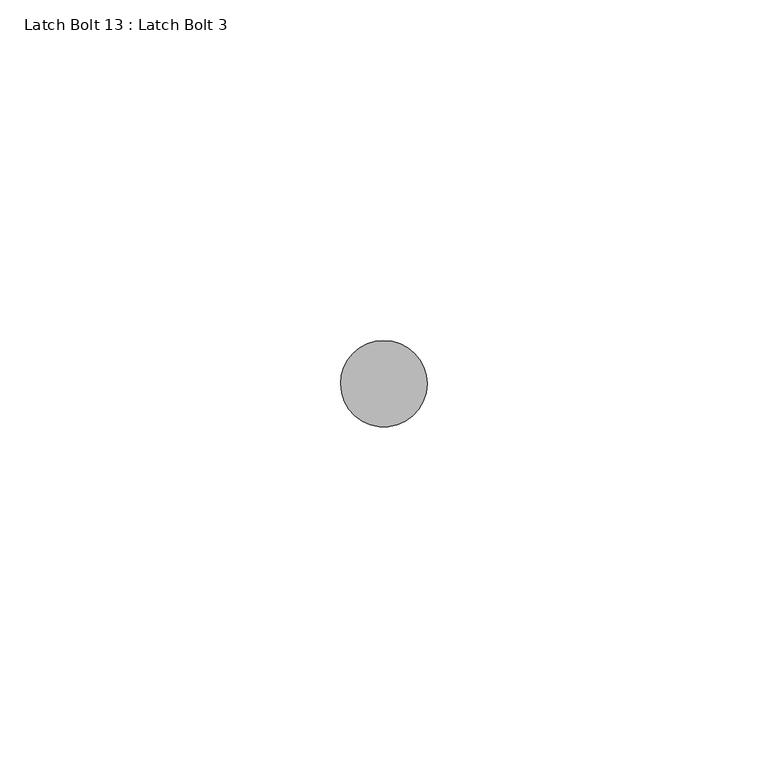
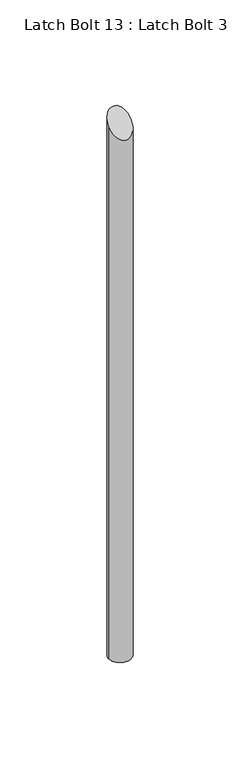
"""IFC4 building model written with IfcOpenShell, lengths in millimetres: proxy geometry, Latch Bolt 13 : Latch Bolt 3."""

import ifcopenshell
import ifcopenshell.guid

model = None  # the IFC model being written
_history = None  # IfcOwnerHistory: only IFC2X3 demands one
_inside = {}  # id of a spatial element -> (the spatial element, [elements in it])
_under = {}  # id of a project, library or spatial element -> (it, [spatial elements below it])
_declared = {}  # id of a project -> (the project, [libraries it declares])
_typed = {}  # id of a type object -> (the type object, [elements of that type])
_made_of = {}  # id of a material, layer set ... -> (it, [elements and type objects made of it])


def new_model(schema):
    """Start an empty IFC model of exactly this schema.

    Asked for "IFC4X3", IfcOpenShell would pick the latest addendum, in which some entities
    have other attributes; the version numbers below select the first issue.
    IFC2X3 requires an IfcOwnerHistory on every rooted entity: one is made here for all.
    """
    global model, _history
    if schema == "IFC4X3":
        model = ifcopenshell.file(schema_version=(4, 3, 0, 0))
    else:
        model = ifcopenshell.file(schema=schema)
    _inside.clear()
    _under.clear()
    _declared.clear()
    _typed.clear()
    _made_of.clear()
    _history = None
    if model.schema == "IFC2X3":
        org = make("IfcOrganization", Name="unknown")
        user = make(
            "IfcPersonAndOrganization",
            ThePerson=make("IfcPerson", FamilyName="unknown"),
            TheOrganization=org,
        )
        app = make(
            "IfcApplication",
            ApplicationDeveloper=org,
            Version="unknown",
            ApplicationFullName="unknown",
            ApplicationIdentifier="unknown",
        )
        _history = make(
            "IfcOwnerHistory",
            OwningUser=user,
            OwningApplication=app,
            ChangeAction="ADDED",
            CreationDate=0,
        )
    return model


def make(cls, **values):
    """One entity of the class cls with the attributes given. An attribute that is None is left unset."""
    return model.create_entity(
        cls, **{name: value for name, value in values.items() if value is not None}
    )


def rooted(cls, **values):
    """An entity with a GlobalId (a new one), such as an element, a storey or a relation."""
    return make(cls, GlobalId=ifcopenshell.guid.new(), OwnerHistory=_history, **values)


def si_unit(unit_type, name, prefix=None):
    """IfcSIUnit, for example si_unit("LENGTHUNIT", "METRE", prefix="MILLI")."""
    return make("IfcSIUnit", UnitType=unit_type, Prefix=prefix, Name=name)


def assignment(units):
    """IfcUnitAssignment: the units of a project."""
    return None if units is None else make("IfcUnitAssignment", Units=units)


def point(xyz):
    """IfcCartesianPoint."""
    return None if xyz is None else make("IfcCartesianPoint", Coordinates=xyz)


def direction(xyz):
    """IfcDirection."""
    return None if xyz is None else make("IfcDirection", DirectionRatios=xyz)


def frame(location, z_axis=None, x_axis=None):
    """IfcAxis2Placement3D, a coordinate frame: its origin and axes. An axis left out is left unset."""
    return make(
        "IfcAxis2Placement3D",
        Location=point(location),
        Axis=direction(z_axis),
        RefDirection=direction(x_axis),
    )


def origin():
    """The frame at (0, 0, 0) with its axes left unset."""
    return frame((0.0, 0.0, 0.0))


def place(relative_to, where):
    """IfcLocalPlacement: puts the frame where relative to a parent placement (None: the world)."""
    return make(
        "IfcLocalPlacement", PlacementRelTo=relative_to, RelativePlacement=where
    )


def context(
    kind, dimensions, precision=None, world=None, true_north=None, identifier=None
):
    """IfcGeometricRepresentationContext, for example the 3D "Model" context."""
    return make(
        "IfcGeometricRepresentationContext",
        ContextIdentifier=identifier,
        ContextType=kind,
        CoordinateSpaceDimension=dimensions,
        Precision=precision,
        WorldCoordinateSystem=world,
        TrueNorth=true_north,
    )


def project(units=None, contexts=None):
    """IfcProject with its units and contexts."""
    return rooted(
        "IfcProject",
        Name="project",
        RepresentationContexts=contexts,
        UnitsInContext=assignment(units),
    )


def spatial(cls, under=None, at=None, **own):
    """A site, building, storey or space (cls), placed at a placement, below another one or the project."""
    s = rooted(cls, ObjectPlacement=at, **own)
    if under is not None:
        _under.setdefault(under.id(), (under, []))[1].append(s)
    return s


def circle_curve(where, radius):
    """IfcCircle in the frame where."""
    return make("IfcCircle", Position=where, Radius=radius)


def ellipse_curve(where, semi_axis1, semi_axis2):
    """IfcEllipse in the frame where."""
    return make(
        "IfcEllipse", Position=where, SemiAxis1=semi_axis1, SemiAxis2=semi_axis2
    )


def shape(context_of_items, identifier, shape_type, items):
    """IfcShapeRepresentation: the items that make up one representation, for example the "Body"."""
    return make(
        "IfcShapeRepresentation",
        ContextOfItems=context_of_items,
        RepresentationIdentifier=identifier,
        RepresentationType=shape_type,
        Items=items,
    )


def source(mapping_origin, context_of_items, identifier, shape_type, items):
    """IfcRepresentationMap: a shape defined once, which mapped items show again and again."""
    return make(
        "IfcRepresentationMap",
        MappingOrigin=mapping_origin,
        MappedRepresentation=shape(context_of_items, identifier, shape_type, items),
    )


def transform(
    local_origin,
    x_axis=None,
    y_axis=None,
    z_axis=None,
    scale=None,
    scale2=None,
    scale3=None,
    uniform=True,
):
    """IfcCartesianTransformationOperator3D, or its non-uniform kind. x_axis, y_axis, z_axis: its Axis1, 2, 3."""
    if uniform:
        return make(
            "IfcCartesianTransformationOperator3D",
            Axis1=direction(x_axis),
            Axis2=direction(y_axis),
            LocalOrigin=point(local_origin),
            Scale=scale,
            Axis3=direction(z_axis),
        )
    return make(
        "IfcCartesianTransformationOperator3DnonUniform",
        Axis1=direction(x_axis),
        Axis2=direction(y_axis),
        LocalOrigin=point(local_origin),
        Scale=scale,
        Axis3=direction(z_axis),
        Scale2=scale2,
        Scale3=scale3,
    )


def mapped(mapping_source, mapping_target):
    """IfcMappedItem: shows the shape of a source again, moved by a transform."""
    return make(
        "IfcMappedItem", MappingSource=mapping_source, MappingTarget=mapping_target
    )


def made_of(thing, what):
    """Note that an element or type object is made of a material, layer set ...; save() writes the relation."""
    if what is not None:
        _made_of.setdefault(what.id(), (what, []))[1].append(thing)
    return thing


def element(
    cls,
    number,
    at=None,
    inside=None,
    cuts=None,
    type_object=None,
    material=None,
    context=None,
    identifier="Body",
    shape_type=None,
    held_by="IfcProductDefinitionShape",
    body=None,
    shapes=None,
    **own,
):
    """One element of the class cls, such as IfcWall. Its Tag is "e" and its number.

    at: its placement. inside: the storey or other place that contains it. cuts: it is an
    opening in that element (IfcRelVoidsElement). A single representation is given by context,
    identifier, shape_type and body (its items); several are given by shapes. held_by: the class
    of the entity that holds the representations. save() writes the other relations.
    """
    e = rooted(cls, Tag="e%d" % number, ObjectPlacement=at, **own)
    if body is not None:
        shapes = [shape(context, identifier, shape_type, body)]
    if shapes is not None:
        e.Representation = make(held_by, Representations=shapes)
    if inside is not None:
        _inside.setdefault(inside.id(), (inside, []))[1].append(e)
    if cuts is not None:
        rooted(
            "IfcRelVoidsElement", RelatingBuildingElement=cuts, RelatedOpeningElement=e
        )
    if type_object is not None:
        _typed.setdefault(type_object.id(), (type_object, []))[1].append(e)
    return made_of(e, material)


def aggregate(whole, parts):
    """IfcRelAggregates: a whole, such as a stair, and the parts it consists of."""
    return rooted("IfcRelAggregates", RelatingObject=whole, RelatedObjects=parts)


def save(model, path):
    """Write the relations noted so far, then the file.

    IfcRelAggregates (storeys below a building ...), IfcRelContainedInSpatialStructure (elements
    in a storey), IfcRelDefinesByType, IfcRelAssociatesMaterial and IfcRelDeclares: one each for
    every whole, place, type object, material and project.
    """
    for whole, parts in _under.values():
        aggregate(whole, parts)
    for where, things in _inside.values():
        rooted(
            "IfcRelContainedInSpatialStructure",
            RelatedElements=things,
            RelatingStructure=where,
        )
    for kind, things in _typed.values():
        rooted("IfcRelDefinesByType", RelatedObjects=things, RelatingType=kind)
    for what, things in _made_of.values():
        rooted("IfcRelAssociatesMaterial", RelatedObjects=things, RelatingMaterial=what)
    for by, libraries in _declared.values():
        rooted("IfcRelDeclares", RelatingContext=by, RelatedDefinitions=libraries)
    model.write(path)


def plane_surface(at):
    """IfcPlane: the flat surface through the origin of the frame at, square to its z axis."""
    return make("IfcPlane", Position=at)


def cylinder_surface(at, radius):
    """IfcCylindricalSurface: all points at the distance radius from the z axis of the frame at."""
    return make("IfcCylindricalSurface", Position=at, Radius=radius)


def advanced_brep(points, edges, surfaces, faces):
    """IfcAdvancedBrep: a solid bounded by faces that lie on surfaces and meet in shared edges.

    An edge is (start, end): straight between two places in points (the first is 0);
    or (start, end, curve); or (start, end, curve, False) where it runs against its curve.
    A face is (place in surfaces, loops), or (place, loops, False) where it looks against
    its surface's normal. A loop lists edges by number (the first is 1), with a minus sign
    where the edge is run from its end to its start. The first loop is the outer one.
    """
    corners = [point(p) for p in points]
    vertices = [make("IfcVertexPoint", VertexGeometry=c) for c in corners]
    made = []
    for start, end, *more in edges:
        made.append(
            make(
                "IfcEdgeCurve",
                EdgeStart=vertices[start],
                EdgeEnd=vertices[end],
                EdgeGeometry=more[0] if more else make("IfcPolyline", Points=[corners[start], corners[end]]),
                SameSense=more[1] if len(more) > 1 else True,
            )
        )
    hull = []
    for where, loops, *sense in faces:
        bounds = []
        for j, loop in enumerate(loops):
            ring = [make("IfcOrientedEdge", EdgeElement=made[abs(k) - 1], Orientation=k > 0) for k in loop]
            bounds.append(
                make(
                    "IfcFaceOuterBound" if j == 0 else "IfcFaceBound",
                    Bound=make("IfcEdgeLoop", EdgeList=ring),
                    Orientation=True,
                )
            )
        hull.append(make("IfcAdvancedFace", Bounds=bounds, FaceSurface=surfaces[where], SameSense=sense[0] if sense else True))
    return make("IfcAdvancedBrep", Outer=make("IfcClosedShell", CfsFaces=hull))


def latch_bolt_13_latch_bolt_3_89fb1f9d(model_context):
    return source(origin(), model_context, "Body", "AdvancedBrep", [
        advanced_brep(
        [(587315.8935739, -535163.4663841, -25.4), (587303.1935739, -535163.4663841, -25.4), (587303.1935739, -535163.4663841, 292.0822144), (587309.5435739, -535157.1163841, 298.4322144), (587315.8935739, -535163.4663841, 292.0822144)],
        [
            (0, 1, circle_curve(frame((587309.5435739, -535163.4663841, -25.4), z_axis=(0.0, 0.0, -1.0), x_axis=(1.0, 0.0, 0.0)), 6.35)),
            (1, 0, circle_curve(frame((587309.5435739, -535163.4663841, -25.4), z_axis=(0.0, 0.0, -1.0), x_axis=(1.0, 0.0, 0.0)), 6.35)),
            (1, 2),
            (2, 3, ellipse_curve(frame((587309.5435739, -535163.4663841, 292.0822144), z_axis=(0.0, 0.7071067811865513, -0.7071067811865438), x_axis=(0.0, 0.7071067811865438, 0.7071067811865512)), 8.9802561, 6.35)),
            (3, 4, ellipse_curve(frame((587309.5435739, -535163.4663841, 292.0822144), z_axis=(0.0, 0.7071067811865513, -0.7071067811865438), x_axis=(0.0, 0.7071067811865438, 0.7071067811865512)), 8.9802561, 6.35)),
            (4, 0),
            (4, 2, ellipse_curve(frame((587309.5435739, -535163.4663841, 292.0822144), z_axis=(0.0, 0.7071067811865513, -0.7071067811865438), x_axis=(0.0, 0.7071067811865438, 0.7071067811865512)), 8.9802561, 6.35)),
        ],
        [
            plane_surface(frame((587315.8935739, -535163.4663841, -25.4), z_axis=(0.0, 0.0, -1.0), x_axis=(0.0, -1.0, 0.0))),
            cylinder_surface(frame((587309.5435739, -535163.4663841, -25.4), z_axis=(0.0, 0.0, 1.0), x_axis=(1.0, 0.0, 0.0)), 6.35),
            plane_surface(frame((587338.1185739, -535157.1163841, 298.4322144), z_axis=(0.0, -0.7071067811865513, 0.7071067811865438), x_axis=(-1.0, 0.0, 0.0))),
        ],
        [
            (0, [[1, 2]]),
            (1, [[-2, 3, 4, 5, 6]]),
            (1, [[-1, -6, 7, -3]]),
            (2, [[-5, -4, -7]]),
        ],
    ),
    ])


if __name__ == "__main__":
    model = new_model("IFC4")
    model_context = context("Model", 3, world=origin())
    ifc_project = project(units=[si_unit("LENGTHUNIT", "METRE", prefix="MILLI")], contexts=[model_context])
    site = spatial("IfcSite", under=ifc_project)
    building = spatial("IfcBuilding", under=site)
    placement = place(None, origin())
    latch_bolt_13_latch_bolt_3_shape = latch_bolt_13_latch_bolt_3_89fb1f9d(model_context)
    element("IfcBuildingElementProxy", 1, Name="Latch Bolt 13 : Latch Bolt 3", ObjectType="Latch Bolt 13 : Latch Bolt 3", at=placement, inside=building, context=model_context, shape_type="MappedRepresentation", body=[
        mapped(latch_bolt_13_latch_bolt_3_shape, transform((0.0, 0.0, 0.0), x_axis=(1.0, 0.0, 0.0), y_axis=(0.0, 1.0, 0.0), z_axis=(0.0, 0.0, 1.0))),
    ])
    save(model, "model.ifc")

# Revit data of these elements
# Element 1 (IfcBuildingElementProxy, "Latch Bolt 13 : Latch Bolt 3")
#   Materials on its faces: "GALV. SLIDE BOLT"
# Materials
#   "GALV. SLIDE BOLT": class "Metal", colour RGB 189 187 185, transparency 0, Description = "Carbon steel", Cost = 0
